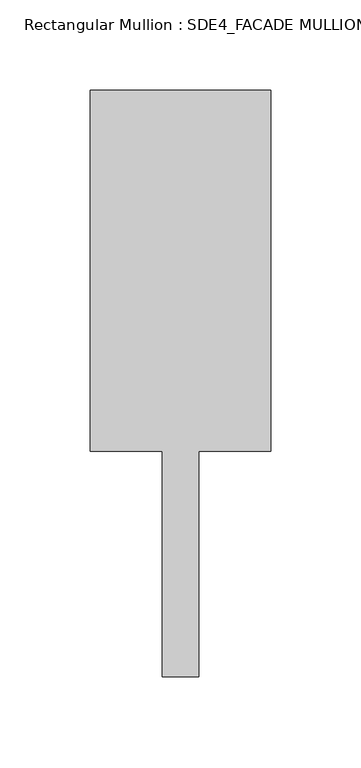
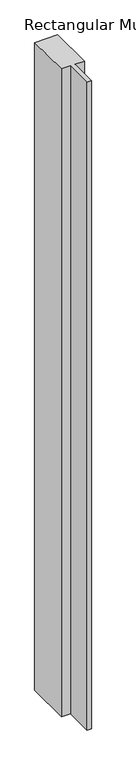
"""IFC4 building model written with IfcOpenShell, lengths in millimetres: member geometry, Rectangular Mullion : SDE4_FACADE MULLION TYPE 2."""

from ifc_helpers import new_model, si_unit, frame, origin, place, context, project, spatial, polyline, outline, extrude, source, transform, mapped, element, save


def rectangular_mullion_sde4_facade_mullion_type_2_5d2f8f9e(model_context):
    return source(origin(), model_context, "Body", "SweptSolid", [
        extrude(outline(polyline([(50.0, 132.5), (50.0, -67.5), (10.0, -67.5), (10.0, -192.5), (-10.0, -192.5), (-10.0, -67.5), (-50.0, -67.5), (-50.0, 132.5), (50.0, 132.5)])), frame((0.0, 0.0, -2970.0), z_axis=(0.0, 0.0, 1.0), x_axis=(1.0, 0.0, 0.0)), (0.0, 0.0, 1.0), 2970.0),
    ])


if __name__ == "__main__":
    model = new_model("IFC4")
    model_context = context("Model", 3, world=origin())
    ifc_project = project(units=[si_unit("LENGTHUNIT", "METRE", prefix="MILLI")], contexts=[model_context])
    site = spatial("IfcSite", under=ifc_project)
    building = spatial("IfcBuilding", under=site)
    placement = place(None, origin())
    rectangular_mullion_sde4_facade_mullion_type_2_shape = rectangular_mullion_sde4_facade_mullion_type_2_5d2f8f9e(model_context)
    element("IfcMember", 1, ObjectType="Rectangular Mullion : SDE4_FACADE MULLION TYPE 2", at=placement, inside=building, context=model_context, shape_type="MappedRepresentation", body=[
        mapped(rectangular_mullion_sde4_facade_mullion_type_2_shape, transform((0.0, 0.0, 0.0), x_axis=(1.0, 0.0, 0.0), y_axis=(0.0, 1.0, 0.0), z_axis=(0.0, 0.0, 1.0))),
    ])
    save(model, "model.ifc")

# Revit data of these elements
# Type "Rectangular Mullion : SDE4_FACADE MULLION TYPE 2"
#   built-in parameter 1007322 = 1.06627 (stored number, unit not read)
#   built-in parameter 1007321 = 0.164042 (stored number, unit not read)
#   built-in parameter 1007320 = 0.164042 (stored number, unit not read)
